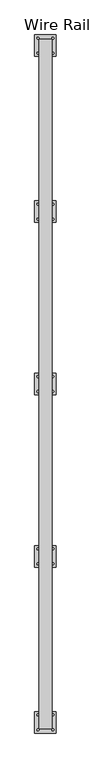
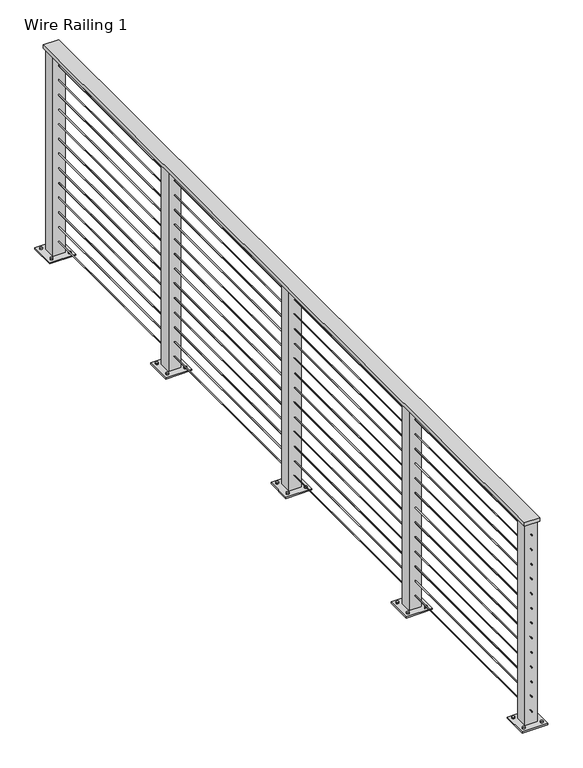
"""IFC4 building model written with IfcOpenShell, lengths in millimetres: railing geometry, Wire Railing 1."""

from ifc_helpers import new_model, si_unit, point, frame, frame_2d, origin, place, context, project, spatial, polyline, circle_curve, trimmed, segment, composite_curve, outline, extrude, source, transform, mapped, element, save


def wire_railing_1_2265859b(model_context):
    return source(origin(), model_context, "Body", "SweptSolid", [
        extrude(outline(polyline([(33170.9291041, 30964.0021048), (33094.7291041, 30964.0021048), (33094.7291041, 35053.4021048), (33170.9291041, 35053.4021048), (33170.9291041, 30964.0021048)])), frame((0.0, 0.0, 270249.65), z_axis=(0.0, 0.0, 1.0), x_axis=(1.0, 0.0, 0.0)), (0.0, 0.0, 1.0), 19.05),
        extrude(outline(composite_curve([segment(trimmed(circle_curve(frame_2d((270190.11875, 33132.8291041)), 2.38125), [point((270190.11875, 33130.4478541))], [point((270190.11875, 33135.2103541))], False, "CARTESIAN"), True, "CONTINUOUS"), segment(trimmed(circle_curve(frame_2d((270190.11875, 33132.8291041)), 2.38125), [point((270190.11875, 33135.2103541))], [point((270190.11875, 33130.4478541))], False, "CARTESIAN"), True, "CONTINUOUS")], self_intersect=False)), frame((0.0, 30964.0021048, 0.0), z_axis=(0.0, 1.0, 0.0), x_axis=(0.0, 0.0, 1.0)), (0.0, 0.0, 1.0), 4089.4),
        extrude(outline(composite_curve([segment(trimmed(circle_curve(frame_2d((270113.91875, 33132.8291041)), 2.38125), [point((270113.91875, 33130.4478541))], [point((270113.91875, 33135.2103541))], False, "CARTESIAN"), True, "CONTINUOUS"), segment(trimmed(circle_curve(frame_2d((270113.91875, 33132.8291041)), 2.38125), [point((270113.91875, 33135.2103541))], [point((270113.91875, 33130.4478541))], False, "CARTESIAN"), True, "CONTINUOUS")], self_intersect=False)), frame((0.0, 30964.0021048, 0.0), z_axis=(0.0, 1.0, 0.0), x_axis=(0.0, 0.0, 1.0)), (0.0, 0.0, 1.0), 4089.4),
        extrude(outline(composite_curve([segment(trimmed(circle_curve(frame_2d((270037.71875, 33132.8291041)), 2.38125), [point((270037.71875, 33130.4478541))], [point((270037.71875, 33135.2103541))], False, "CARTESIAN"), True, "CONTINUOUS"), segment(trimmed(circle_curve(frame_2d((270037.71875, 33132.8291041)), 2.38125), [point((270037.71875, 33135.2103541))], [point((270037.71875, 33130.4478541))], False, "CARTESIAN"), True, "CONTINUOUS")], self_intersect=False)), frame((0.0, 30964.0021048, 0.0), z_axis=(0.0, 1.0, 0.0), x_axis=(0.0, 0.0, 1.0)), (0.0, 0.0, 1.0), 4089.4),
        extrude(outline(composite_curve([segment(trimmed(circle_curve(frame_2d((269961.51875, 33132.8291041)), 2.38125), [point((269961.51875, 33130.4478541))], [point((269961.51875, 33135.2103541))], False, "CARTESIAN"), True, "CONTINUOUS"), segment(trimmed(circle_curve(frame_2d((269961.51875, 33132.8291041)), 2.38125), [point((269961.51875, 33135.2103541))], [point((269961.51875, 33130.4478541))], False, "CARTESIAN"), True, "CONTINUOUS")], self_intersect=False)), frame((0.0, 30964.0021048, 0.0), z_axis=(0.0, 1.0, 0.0), x_axis=(0.0, 0.0, 1.0)), (0.0, 0.0, 1.0), 4089.4),
        extrude(outline(composite_curve([segment(trimmed(circle_curve(frame_2d((269885.31875, 33132.8291041)), 2.38125), [point((269885.31875, 33130.4478541))], [point((269885.31875, 33135.2103541))], False, "CARTESIAN"), True, "CONTINUOUS"), segment(trimmed(circle_curve(frame_2d((269885.31875, 33132.8291041)), 2.38125), [point((269885.31875, 33135.2103541))], [point((269885.31875, 33130.4478541))], False, "CARTESIAN"), True, "CONTINUOUS")], self_intersect=False)), frame((0.0, 30964.0021048, 0.0), z_axis=(0.0, 1.0, 0.0), x_axis=(0.0, 0.0, 1.0)), (0.0, 0.0, 1.0), 4089.4),
        extrude(outline(composite_curve([segment(trimmed(circle_curve(frame_2d((269809.11875, 33132.8291041)), 2.38125), [point((269809.11875, 33130.4478541))], [point((269809.11875, 33135.2103541))], False, "CARTESIAN"), True, "CONTINUOUS"), segment(trimmed(circle_curve(frame_2d((269809.11875, 33132.8291041)), 2.38125), [point((269809.11875, 33135.2103541))], [point((269809.11875, 33130.4478541))], False, "CARTESIAN"), True, "CONTINUOUS")], self_intersect=False)), frame((0.0, 30964.0021048, 0.0), z_axis=(0.0, 1.0, 0.0), x_axis=(0.0, 0.0, 1.0)), (0.0, 0.0, 1.0), 4089.4),
        extrude(outline(composite_curve([segment(trimmed(circle_curve(frame_2d((269732.91875, 33132.8291041)), 2.38125), [point((269732.91875, 33130.4478541))], [point((269732.91875, 33135.2103541))], False, "CARTESIAN"), True, "CONTINUOUS"), segment(trimmed(circle_curve(frame_2d((269732.91875, 33132.8291041)), 2.38125), [point((269732.91875, 33135.2103541))], [point((269732.91875, 33130.4478541))], False, "CARTESIAN"), True, "CONTINUOUS")], self_intersect=False)), frame((0.0, 30964.0021048, 0.0), z_axis=(0.0, 1.0, 0.0), x_axis=(0.0, 0.0, 1.0)), (0.0, 0.0, 1.0), 4089.4),
        extrude(outline(composite_curve([segment(trimmed(circle_curve(frame_2d((269656.71875, 33132.8291041)), 2.38125), [point((269656.71875, 33130.4478541))], [point((269656.71875, 33135.2103541))], False, "CARTESIAN"), True, "CONTINUOUS"), segment(trimmed(circle_curve(frame_2d((269656.71875, 33132.8291041)), 2.38125), [point((269656.71875, 33135.2103541))], [point((269656.71875, 33130.4478541))], False, "CARTESIAN"), True, "CONTINUOUS")], self_intersect=False)), frame((0.0, 30964.0021048, 0.0), z_axis=(0.0, 1.0, 0.0), x_axis=(0.0, 0.0, 1.0)), (0.0, 0.0, 1.0), 4089.4),
        extrude(outline(composite_curve([segment(trimmed(circle_curve(frame_2d((269580.51875, 33132.8291041)), 2.38125), [point((269580.51875, 33130.4478541))], [point((269580.51875, 33135.2103541))], False, "CARTESIAN"), True, "CONTINUOUS"), segment(trimmed(circle_curve(frame_2d((269580.51875, 33132.8291041)), 2.38125), [point((269580.51875, 33135.2103541))], [point((269580.51875, 33130.4478541))], False, "CARTESIAN"), True, "CONTINUOUS")], self_intersect=False)), frame((0.0, 30964.0021048, 0.0), z_axis=(0.0, 1.0, 0.0), x_axis=(0.0, 0.0, 1.0)), (0.0, 0.0, 1.0), 4089.4),
        extrude(outline(composite_curve([segment(trimmed(circle_curve(frame_2d((269504.31875, 33132.8291041)), 2.38125), [point((269504.31875, 33130.4478541))], [point((269504.31875, 33135.2103541))], False, "CARTESIAN"), True, "CONTINUOUS"), segment(trimmed(circle_curve(frame_2d((269504.31875, 33132.8291041)), 2.38125), [point((269504.31875, 33135.2103541))], [point((269504.31875, 33130.4478541))], False, "CARTESIAN"), True, "CONTINUOUS")], self_intersect=False)), frame((0.0, 30964.0021048, 0.0), z_axis=(0.0, 1.0, 0.0), x_axis=(0.0, 0.0, 1.0)), (0.0, 0.0, 1.0), 4089.4),
        extrude(outline(composite_curve([segment(trimmed(circle_curve(frame_2d((269428.11875, 33132.8291041)), 2.38125), [point((269428.11875, 33130.4478541))], [point((269428.11875, 33135.2103541))], False, "CARTESIAN"), True, "CONTINUOUS"), segment(trimmed(circle_curve(frame_2d((269428.11875, 33132.8291041)), 2.38125), [point((269428.11875, 33135.2103541))], [point((269428.11875, 33130.4478541))], False, "CARTESIAN"), True, "CONTINUOUS")], self_intersect=False)), frame((0.0, 30964.0021048, 0.0), z_axis=(0.0, 1.0, 0.0), x_axis=(0.0, 0.0, 1.0)), (0.0, 0.0, 1.0), 4089.4),
        extrude(outline(composite_curve([segment(trimmed(circle_curve(frame_2d((269351.91875, 33132.8291041)), 2.38125), [point((269351.91875, 33130.4478541))], [point((269351.91875, 33135.2103541))], False, "CARTESIAN"), True, "CONTINUOUS"), segment(trimmed(circle_curve(frame_2d((269351.91875, 33132.8291041)), 2.38125), [point((269351.91875, 33135.2103541))], [point((269351.91875, 33130.4478541))], False, "CARTESIAN"), True, "CONTINUOUS")], self_intersect=False)), frame((0.0, 30964.0021048, 0.0), z_axis=(0.0, 1.0, 0.0), x_axis=(0.0, 0.0, 1.0)), (0.0, 0.0, 1.0), 4089.4),
        extrude(outline(composite_curve([segment(trimmed(circle_curve(frame_2d((269275.71875, 33132.8291041)), 2.38125), [point((269275.71875, 33130.4478541))], [point((269275.71875, 33135.2103541))], False, "CARTESIAN"), True, "CONTINUOUS"), segment(trimmed(circle_curve(frame_2d((269275.71875, 33132.8291041)), 2.38125), [point((269275.71875, 33135.2103541))], [point((269275.71875, 33130.4478541))], False, "CARTESIAN"), True, "CONTINUOUS")], self_intersect=False)), frame((0.0, 30964.0021048, 0.0), z_axis=(0.0, 1.0, 0.0), x_axis=(0.0, 0.0, 1.0)), (0.0, 0.0, 1.0), 4089.4),
        extrude(outline(composite_curve([segment(trimmed(circle_curve(frame_2d((33177.2791041, 33986.6021048)), 6.35), [point((33183.6291041, 33986.6021048))], [point((33170.9291041, 33986.6021048))], False, "CARTESIAN"), True, "CONTINUOUS"), segment(trimmed(circle_curve(frame_2d((33177.2791041, 33986.6021048)), 6.35), [point((33170.9291041, 33986.6021048))], [point((33183.6291041, 33986.6021048))], False, "CARTESIAN"), True, "CONTINUOUS")], self_intersect=False)), frame((0.0, 0.0, 269201.9), z_axis=(0.0, 0.0, 1.0), x_axis=(1.0, 0.0, 0.0)), (0.0, 0.0, 1.0), 12.7),
        extrude(outline(composite_curve([segment(trimmed(circle_curve(frame_2d((33088.3791041, 33986.6021048)), 6.35), [point((33094.7291041, 33986.6021048))], [point((33082.0291041, 33986.6021048))], False, "CARTESIAN"), True, "CONTINUOUS"), segment(trimmed(circle_curve(frame_2d((33088.3791041, 33986.6021048)), 6.35), [point((33082.0291041, 33986.6021048))], [point((33094.7291041, 33986.6021048))], False, "CARTESIAN"), True, "CONTINUOUS")], self_intersect=False)), frame((0.0, 0.0, 269201.9), z_axis=(0.0, 0.0, 1.0), x_axis=(1.0, 0.0, 0.0)), (0.0, 0.0, 1.0), 12.7),
        extrude(outline(composite_curve([segment(trimmed(circle_curve(frame_2d((33177.2791041, 34075.5021048)), 6.35), [point((33183.6291041, 34075.5021048))], [point((33170.9291041, 34075.5021048))], False, "CARTESIAN"), True, "CONTINUOUS"), segment(trimmed(circle_curve(frame_2d((33177.2791041, 34075.5021048)), 6.35), [point((33170.9291041, 34075.5021048))], [point((33183.6291041, 34075.5021048))], False, "CARTESIAN"), True, "CONTINUOUS")], self_intersect=False)), frame((0.0, 0.0, 269201.9), z_axis=(0.0, 0.0, 1.0), x_axis=(1.0, 0.0, 0.0)), (0.0, 0.0, 1.0), 12.7),
        extrude(outline(composite_curve([segment(trimmed(circle_curve(frame_2d((33088.3791041, 34075.5021048)), 6.35), [point((33094.7291041, 34075.5021048))], [point((33082.0291041, 34075.5021048))], False, "CARTESIAN"), True, "CONTINUOUS"), segment(trimmed(circle_curve(frame_2d((33088.3791041, 34075.5021048)), 6.35), [point((33082.0291041, 34075.5021048))], [point((33094.7291041, 34075.5021048))], False, "CARTESIAN"), True, "CONTINUOUS")], self_intersect=False)), frame((0.0, 0.0, 269201.9), z_axis=(0.0, 0.0, 1.0), x_axis=(1.0, 0.0, 0.0)), (0.0, 0.0, 1.0), 12.7),
        extrude(outline(polyline([(33069.3291041, 33967.5521048), (33069.3291041, 34094.5521048), (33196.3291041, 34094.5521048), (33196.3291041, 33967.5521048), (33069.3291041, 33967.5521048)])), frame((0.0, 0.0, 269201.9), z_axis=(0.0, 0.0, 1.0), x_axis=(1.0, 0.0, 0.0)), (0.0, 0.0, 1.0), 6.35),
        extrude(outline(polyline([(33102.6666041, 34000.8896048), (33102.6666041, 34061.2146048), (33162.9916041, 34061.2146048), (33162.9916041, 34000.8896048), (33102.6666041, 34000.8896048)]), holes=[polyline([(33109.0166041, 34007.2396048), (33156.6416041, 34007.2396048), (33156.6416041, 34054.8646048), (33109.0166041, 34054.8646048), (33109.0166041, 34007.2396048)])]), frame((0.0, 0.0, 269201.9), z_axis=(0.0, 0.0, 1.0), x_axis=(1.0, 0.0, 0.0)), (0.0, 0.0, 1.0), 1047.75),
        extrude(outline(composite_curve([segment(trimmed(circle_curve(frame_2d((33177.2791041, 32964.2521048)), 6.35), [point((33183.6291041, 32964.2521048))], [point((33170.9291041, 32964.2521048))], False, "CARTESIAN"), True, "CONTINUOUS"), segment(trimmed(circle_curve(frame_2d((33177.2791041, 32964.2521048)), 6.35), [point((33170.9291041, 32964.2521048))], [point((33183.6291041, 32964.2521048))], False, "CARTESIAN"), True, "CONTINUOUS")], self_intersect=False)), frame((0.0, 0.0, 269201.9), z_axis=(0.0, 0.0, 1.0), x_axis=(1.0, 0.0, 0.0)), (0.0, 0.0, 1.0), 12.7),
        extrude(outline(composite_curve([segment(trimmed(circle_curve(frame_2d((33088.3791041, 32964.2521048)), 6.35), [point((33094.7291041, 32964.2521048))], [point((33082.0291041, 32964.2521048))], False, "CARTESIAN"), True, "CONTINUOUS"), segment(trimmed(circle_curve(frame_2d((33088.3791041, 32964.2521048)), 6.35), [point((33082.0291041, 32964.2521048))], [point((33094.7291041, 32964.2521048))], False, "CARTESIAN"), True, "CONTINUOUS")], self_intersect=False)), frame((0.0, 0.0, 269201.9), z_axis=(0.0, 0.0, 1.0), x_axis=(1.0, 0.0, 0.0)), (0.0, 0.0, 1.0), 12.7),
        extrude(outline(composite_curve([segment(trimmed(circle_curve(frame_2d((33177.2791041, 33053.1521048)), 6.35), [point((33183.6291041, 33053.1521048))], [point((33170.9291041, 33053.1521048))], False, "CARTESIAN"), True, "CONTINUOUS"), segment(trimmed(circle_curve(frame_2d((33177.2791041, 33053.1521048)), 6.35), [point((33170.9291041, 33053.1521048))], [point((33183.6291041, 33053.1521048))], False, "CARTESIAN"), True, "CONTINUOUS")], self_intersect=False)), frame((0.0, 0.0, 269201.9), z_axis=(0.0, 0.0, 1.0), x_axis=(1.0, 0.0, 0.0)), (0.0, 0.0, 1.0), 12.7),
        extrude(outline(composite_curve([segment(trimmed(circle_curve(frame_2d((33088.3791041, 33053.1521048)), 6.35), [point((33094.7291041, 33053.1521048))], [point((33082.0291041, 33053.1521048))], False, "CARTESIAN"), True, "CONTINUOUS"), segment(trimmed(circle_curve(frame_2d((33088.3791041, 33053.1521048)), 6.35), [point((33082.0291041, 33053.1521048))], [point((33094.7291041, 33053.1521048))], False, "CARTESIAN"), True, "CONTINUOUS")], self_intersect=False)), frame((0.0, 0.0, 269201.9), z_axis=(0.0, 0.0, 1.0), x_axis=(1.0, 0.0, 0.0)), (0.0, 0.0, 1.0), 12.7),
        extrude(outline(polyline([(33069.3291041, 32945.2021048), (33069.3291041, 33072.2021048), (33196.3291041, 33072.2021048), (33196.3291041, 32945.2021048), (33069.3291041, 32945.2021048)])), frame((0.0, 0.0, 269201.9), z_axis=(0.0, 0.0, 1.0), x_axis=(1.0, 0.0, 0.0)), (0.0, 0.0, 1.0), 6.35),
        extrude(outline(polyline([(33102.6666041, 32978.5396048), (33102.6666041, 33038.8646048), (33162.9916041, 33038.8646048), (33162.9916041, 32978.5396048), (33102.6666041, 32978.5396048)]), holes=[polyline([(33109.0166041, 32984.8896048), (33156.6416041, 32984.8896048), (33156.6416041, 33032.5146048), (33109.0166041, 33032.5146048), (33109.0166041, 32984.8896048)])]), frame((0.0, 0.0, 269201.9), z_axis=(0.0, 0.0, 1.0), x_axis=(1.0, 0.0, 0.0)), (0.0, 0.0, 1.0), 1047.75),
        extrude(outline(composite_curve([segment(trimmed(circle_curve(frame_2d((33177.2791041, 31941.9021048)), 6.35), [point((33183.6291041, 31941.9021048))], [point((33170.9291041, 31941.9021048))], False, "CARTESIAN"), True, "CONTINUOUS"), segment(trimmed(circle_curve(frame_2d((33177.2791041, 31941.9021048)), 6.35), [point((33170.9291041, 31941.9021048))], [point((33183.6291041, 31941.9021048))], False, "CARTESIAN"), True, "CONTINUOUS")], self_intersect=False)), frame((0.0, 0.0, 269201.9), z_axis=(0.0, 0.0, 1.0), x_axis=(1.0, 0.0, 0.0)), (0.0, 0.0, 1.0), 12.7),
        extrude(outline(composite_curve([segment(trimmed(circle_curve(frame_2d((33088.3791041, 31941.9021048)), 6.35), [point((33094.7291041, 31941.9021048))], [point((33082.0291041, 31941.9021048))], False, "CARTESIAN"), True, "CONTINUOUS"), segment(trimmed(circle_curve(frame_2d((33088.3791041, 31941.9021048)), 6.35), [point((33082.0291041, 31941.9021048))], [point((33094.7291041, 31941.9021048))], False, "CARTESIAN"), True, "CONTINUOUS")], self_intersect=False)), frame((0.0, 0.0, 269201.9), z_axis=(0.0, 0.0, 1.0), x_axis=(1.0, 0.0, 0.0)), (0.0, 0.0, 1.0), 12.7),
        extrude(outline(composite_curve([segment(trimmed(circle_curve(frame_2d((33177.2791041, 32030.8021048)), 6.35), [point((33183.6291041, 32030.8021048))], [point((33170.9291041, 32030.8021048))], False, "CARTESIAN"), True, "CONTINUOUS"), segment(trimmed(circle_curve(frame_2d((33177.2791041, 32030.8021048)), 6.35), [point((33170.9291041, 32030.8021048))], [point((33183.6291041, 32030.8021048))], False, "CARTESIAN"), True, "CONTINUOUS")], self_intersect=False)), frame((0.0, 0.0, 269201.9), z_axis=(0.0, 0.0, 1.0), x_axis=(1.0, 0.0, 0.0)), (0.0, 0.0, 1.0), 12.7),
        extrude(outline(composite_curve([segment(trimmed(circle_curve(frame_2d((33088.3791041, 32030.8021048)), 6.35), [point((33094.7291041, 32030.8021048))], [point((33082.0291041, 32030.8021048))], False, "CARTESIAN"), True, "CONTINUOUS"), segment(trimmed(circle_curve(frame_2d((33088.3791041, 32030.8021048)), 6.35), [point((33082.0291041, 32030.8021048))], [point((33094.7291041, 32030.8021048))], False, "CARTESIAN"), True, "CONTINUOUS")], self_intersect=False)), frame((0.0, 0.0, 269201.9), z_axis=(0.0, 0.0, 1.0), x_axis=(1.0, 0.0, 0.0)), (0.0, 0.0, 1.0), 12.7),
        extrude(outline(polyline([(33069.3291041, 31922.8521048), (33069.3291041, 32049.8521048), (33196.3291041, 32049.8521048), (33196.3291041, 31922.8521048), (33069.3291041, 31922.8521048)])), frame((0.0, 0.0, 269201.9), z_axis=(0.0, 0.0, 1.0), x_axis=(1.0, 0.0, 0.0)), (0.0, 0.0, 1.0), 6.35),
        extrude(outline(polyline([(33102.6666041, 31956.1896048), (33102.6666041, 32016.5146048), (33162.9916041, 32016.5146048), (33162.9916041, 31956.1896048), (33102.6666041, 31956.1896048)]), holes=[polyline([(33109.0166041, 31962.5396048), (33156.6416041, 31962.5396048), (33156.6416041, 32010.1646048), (33109.0166041, 32010.1646048), (33109.0166041, 31962.5396048)])]), frame((0.0, 0.0, 269201.9), z_axis=(0.0, 0.0, 1.0), x_axis=(1.0, 0.0, 0.0)), (0.0, 0.0, 1.0), 1047.75),
        extrude(outline(composite_curve([segment(trimmed(circle_curve(frame_2d((33177.2791041, 34970.8521048)), 6.35), [point((33183.6291041, 34970.8521048))], [point((33170.9291041, 34970.8521048))], False, "CARTESIAN"), True, "CONTINUOUS"), segment(trimmed(circle_curve(frame_2d((33177.2791041, 34970.8521048)), 6.35), [point((33170.9291041, 34970.8521048))], [point((33183.6291041, 34970.8521048))], False, "CARTESIAN"), True, "CONTINUOUS")], self_intersect=False)), frame((0.0, 0.0, 269201.9), z_axis=(0.0, 0.0, 1.0), x_axis=(1.0, 0.0, 0.0)), (0.0, 0.0, 1.0), 12.7),
        extrude(outline(composite_curve([segment(trimmed(circle_curve(frame_2d((33088.3791041, 34970.8521048)), 6.35), [point((33094.7291041, 34970.8521048))], [point((33082.0291041, 34970.8521048))], False, "CARTESIAN"), True, "CONTINUOUS"), segment(trimmed(circle_curve(frame_2d((33088.3791041, 34970.8521048)), 6.35), [point((33082.0291041, 34970.8521048))], [point((33094.7291041, 34970.8521048))], False, "CARTESIAN"), True, "CONTINUOUS")], self_intersect=False)), frame((0.0, 0.0, 269201.9), z_axis=(0.0, 0.0, 1.0), x_axis=(1.0, 0.0, 0.0)), (0.0, 0.0, 1.0), 12.7),
        extrude(outline(composite_curve([segment(trimmed(circle_curve(frame_2d((33177.2791041, 35059.7521048)), 6.35), [point((33183.6291041, 35059.7521048))], [point((33170.9291041, 35059.7521048))], False, "CARTESIAN"), True, "CONTINUOUS"), segment(trimmed(circle_curve(frame_2d((33177.2791041, 35059.7521048)), 6.35), [point((33170.9291041, 35059.7521048))], [point((33183.6291041, 35059.7521048))], False, "CARTESIAN"), True, "CONTINUOUS")], self_intersect=False)), frame((0.0, 0.0, 269201.9), z_axis=(0.0, 0.0, 1.0), x_axis=(1.0, 0.0, 0.0)), (0.0, 0.0, 1.0), 12.7),
        extrude(outline(composite_curve([segment(trimmed(circle_curve(frame_2d((33088.3791041, 35059.7521048)), 6.35), [point((33094.7291041, 35059.7521048))], [point((33082.0291041, 35059.7521048))], False, "CARTESIAN"), True, "CONTINUOUS"), segment(trimmed(circle_curve(frame_2d((33088.3791041, 35059.7521048)), 6.35), [point((33082.0291041, 35059.7521048))], [point((33094.7291041, 35059.7521048))], False, "CARTESIAN"), True, "CONTINUOUS")], self_intersect=False)), frame((0.0, 0.0, 269201.9), z_axis=(0.0, 0.0, 1.0), x_axis=(1.0, 0.0, 0.0)), (0.0, 0.0, 1.0), 12.7),
        extrude(outline(polyline([(33069.3291041, 34951.8021048), (33069.3291041, 35078.8021048), (33196.3291041, 35078.8021048), (33196.3291041, 34951.8021048), (33069.3291041, 34951.8021048)])), frame((0.0, 0.0, 269201.9), z_axis=(0.0, 0.0, 1.0), x_axis=(1.0, 0.0, 0.0)), (0.0, 0.0, 1.0), 6.35),
        extrude(outline(polyline([(33102.6666041, 34985.1396048), (33102.6666041, 35045.4646048), (33162.9916041, 35045.4646048), (33162.9916041, 34985.1396048), (33102.6666041, 34985.1396048)]), holes=[polyline([(33109.0166041, 34991.4896048), (33156.6416041, 34991.4896048), (33156.6416041, 35039.1146048), (33109.0166041, 35039.1146048), (33109.0166041, 34991.4896048)])]), frame((0.0, 0.0, 269201.9), z_axis=(0.0, 0.0, 1.0), x_axis=(1.0, 0.0, 0.0)), (0.0, 0.0, 1.0), 1047.75),
        extrude(outline(composite_curve([segment(trimmed(circle_curve(frame_2d((33177.2791041, 30957.6521048)), 6.35), [point((33183.6291041, 30957.6521048))], [point((33170.9291041, 30957.6521048))], False, "CARTESIAN"), True, "CONTINUOUS"), segment(trimmed(circle_curve(frame_2d((33177.2791041, 30957.6521048)), 6.35), [point((33170.9291041, 30957.6521048))], [point((33183.6291041, 30957.6521048))], False, "CARTESIAN"), True, "CONTINUOUS")], self_intersect=False)), frame((0.0, 0.0, 269201.9), z_axis=(0.0, 0.0, 1.0), x_axis=(1.0, 0.0, 0.0)), (0.0, 0.0, 1.0), 12.7),
        extrude(outline(composite_curve([segment(trimmed(circle_curve(frame_2d((33088.3791041, 30957.6521048)), 6.35), [point((33094.7291041, 30957.6521048))], [point((33082.0291041, 30957.6521048))], False, "CARTESIAN"), True, "CONTINUOUS"), segment(trimmed(circle_curve(frame_2d((33088.3791041, 30957.6521048)), 6.35), [point((33082.0291041, 30957.6521048))], [point((33094.7291041, 30957.6521048))], False, "CARTESIAN"), True, "CONTINUOUS")], self_intersect=False)), frame((0.0, 0.0, 269201.9), z_axis=(0.0, 0.0, 1.0), x_axis=(1.0, 0.0, 0.0)), (0.0, 0.0, 1.0), 12.7),
        extrude(outline(composite_curve([segment(trimmed(circle_curve(frame_2d((33177.2791041, 31046.5521048)), 6.35), [point((33183.6291041, 31046.5521048))], [point((33170.9291041, 31046.5521048))], False, "CARTESIAN"), True, "CONTINUOUS"), segment(trimmed(circle_curve(frame_2d((33177.2791041, 31046.5521048)), 6.35), [point((33170.9291041, 31046.5521048))], [point((33183.6291041, 31046.5521048))], False, "CARTESIAN"), True, "CONTINUOUS")], self_intersect=False)), frame((0.0, 0.0, 269201.9), z_axis=(0.0, 0.0, 1.0), x_axis=(1.0, 0.0, 0.0)), (0.0, 0.0, 1.0), 12.7),
        extrude(outline(composite_curve([segment(trimmed(circle_curve(frame_2d((33088.3791041, 31046.5521048)), 6.35), [point((33094.7291041, 31046.5521048))], [point((33082.0291041, 31046.5521048))], False, "CARTESIAN"), True, "CONTINUOUS"), segment(trimmed(circle_curve(frame_2d((33088.3791041, 31046.5521048)), 6.35), [point((33082.0291041, 31046.5521048))], [point((33094.7291041, 31046.5521048))], False, "CARTESIAN"), True, "CONTINUOUS")], self_intersect=False)), frame((0.0, 0.0, 269201.9), z_axis=(0.0, 0.0, 1.0), x_axis=(1.0, 0.0, 0.0)), (0.0, 0.0, 1.0), 12.7),
        extrude(outline(polyline([(33069.3291041, 30938.6021048), (33069.3291041, 31065.6021048), (33196.3291041, 31065.6021048), (33196.3291041, 30938.6021048), (33069.3291041, 30938.6021048)])), frame((0.0, 0.0, 269201.9), z_axis=(0.0, 0.0, 1.0), x_axis=(1.0, 0.0, 0.0)), (0.0, 0.0, 1.0), 6.35),
        extrude(outline(polyline([(33102.6666041, 30971.9396048), (33102.6666041, 31032.2646048), (33162.9916041, 31032.2646048), (33162.9916041, 30971.9396048), (33102.6666041, 30971.9396048)]), holes=[polyline([(33109.0166041, 30978.2896048), (33156.6416041, 30978.2896048), (33156.6416041, 31025.9146048), (33109.0166041, 31025.9146048), (33109.0166041, 30978.2896048)])]), frame((0.0, 0.0, 269201.9), z_axis=(0.0, 0.0, 1.0), x_axis=(1.0, 0.0, 0.0)), (0.0, 0.0, 1.0), 1047.75),
    ])


if __name__ == "__main__":
    model = new_model("IFC4")
    model_context = context("Model", 3, world=origin())
    ifc_project = project(units=[si_unit("LENGTHUNIT", "METRE", prefix="MILLI")], contexts=[model_context])
    site = spatial("IfcSite", under=ifc_project)
    building = spatial("IfcBuilding", under=site)
    placement = place(None, origin())
    wire_railing_1_shape = wire_railing_1_2265859b(model_context)
    element("IfcRailing", 1, ObjectType="Wire Railing 1", at=placement, inside=building, context=model_context, shape_type="MappedRepresentation", body=[
        mapped(wire_railing_1_shape, transform((0.0, 0.0, 0.0), x_axis=(1.0, 0.0, 0.0), y_axis=(0.0, 1.0, 0.0), z_axis=(0.0, 0.0, 1.0))),
    ])
    save(model, "model.ifc")

# Revit data of these elements
# Element 1 (IfcRailing, "Wire Railing 1")
#   Materials on its faces: "WIRE RAILING"
# Materials
#   "WIRE RAILING": class "Metal", colour RGB 244 244 244, transparency 0, Manufacturer = "Kawneer", URL = "http://www.kawneer.com/kawneer/north_america/en/home.asp", Cost = 0
